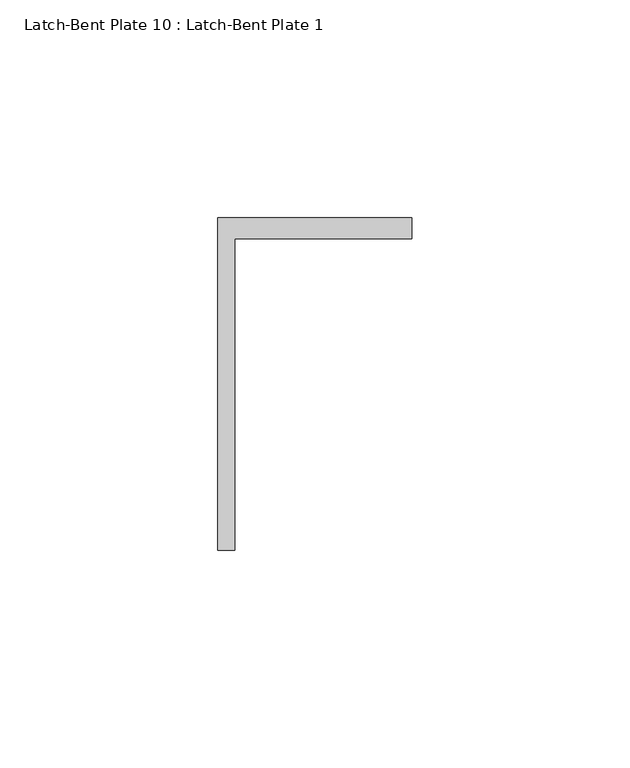
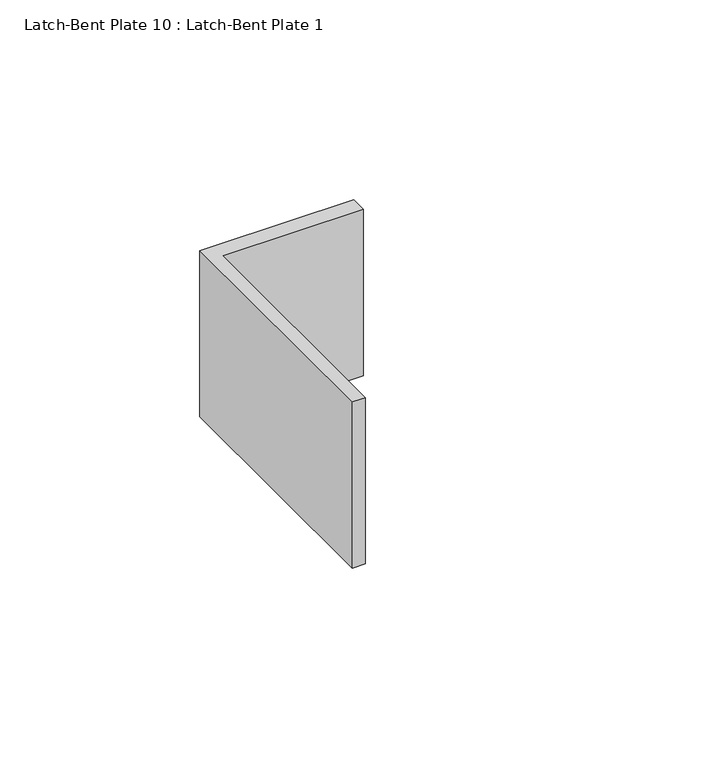
"""IFC4 building model written with IfcOpenShell, lengths in millimetres: proxy geometry, Latch-Bent Plate 10 : Latch-Bent Plate 1."""

from ifc_helpers import new_model, si_unit, frame, origin, place, context, project, spatial, polyline, outline, extrude, source, transform, mapped, element, save


def latch_bent_plate_10_latch_bent_plate_1_12525892(model_context):
    return source(origin(), model_context, "Body", "SweptSolid", [
        extrude(outline(polyline([(587327.0060739, -532883.8163841), (587366.6808739, -532883.8163841), (587366.6808739, -532888.5788841), (587326.1141748, -532888.5788841), (587326.1141748, -532960.0163841), (587322.2435739, -532960.0163841), (587322.2435739, -532883.8163841), (587327.0060739, -532883.8163841)])), frame((0.0, 0.0, 1041.4), z_axis=(0.0, 0.0, 1.0), x_axis=(1.0, 0.0, 0.0)), (0.0, 0.0, 1.0), 50.8),
    ])


if __name__ == "__main__":
    model = new_model("IFC4")
    model_context = context("Model", 3, world=origin())
    ifc_project = project(units=[si_unit("LENGTHUNIT", "METRE", prefix="MILLI")], contexts=[model_context])
    site = spatial("IfcSite", under=ifc_project)
    building = spatial("IfcBuilding", under=site)
    placement = place(None, origin())
    latch_bent_plate_10_latch_bent_plate_1_shape = latch_bent_plate_10_latch_bent_plate_1_12525892(model_context)
    element("IfcBuildingElementProxy", 1, Name="Latch-Bent Plate 10 : Latch-Bent Plate 1", ObjectType="Latch-Bent Plate 10 : Latch-Bent Plate 1", at=placement, inside=building, context=model_context, shape_type="MappedRepresentation", body=[
        mapped(latch_bent_plate_10_latch_bent_plate_1_shape, transform((0.0, 0.0, 0.0), x_axis=(1.0, 0.0, 0.0), y_axis=(0.0, 1.0, 0.0), z_axis=(0.0, 0.0, 1.0))),
    ])
    save(model, "model.ifc")

# Revit data of these elements
# Element 1 (IfcBuildingElementProxy, "Latch-Bent Plate 10 : Latch-Bent Plate 1")
#   Materials on its faces: "GALV. GATE LATCH"
# Materials
#   "GALV. GATE LATCH": class "Metal", colour RGB 189 187 185, transparency 0, Description = "Carbon steel", Cost = 0
